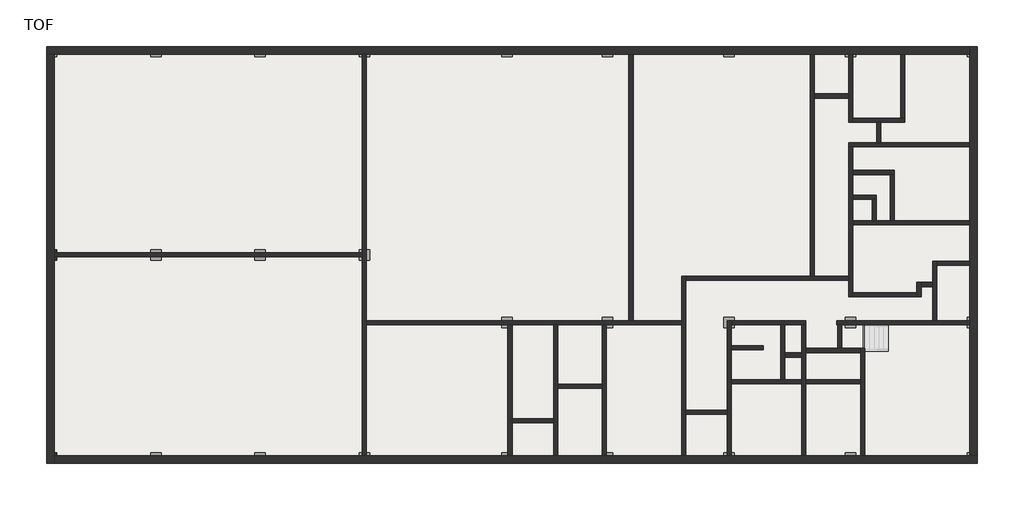
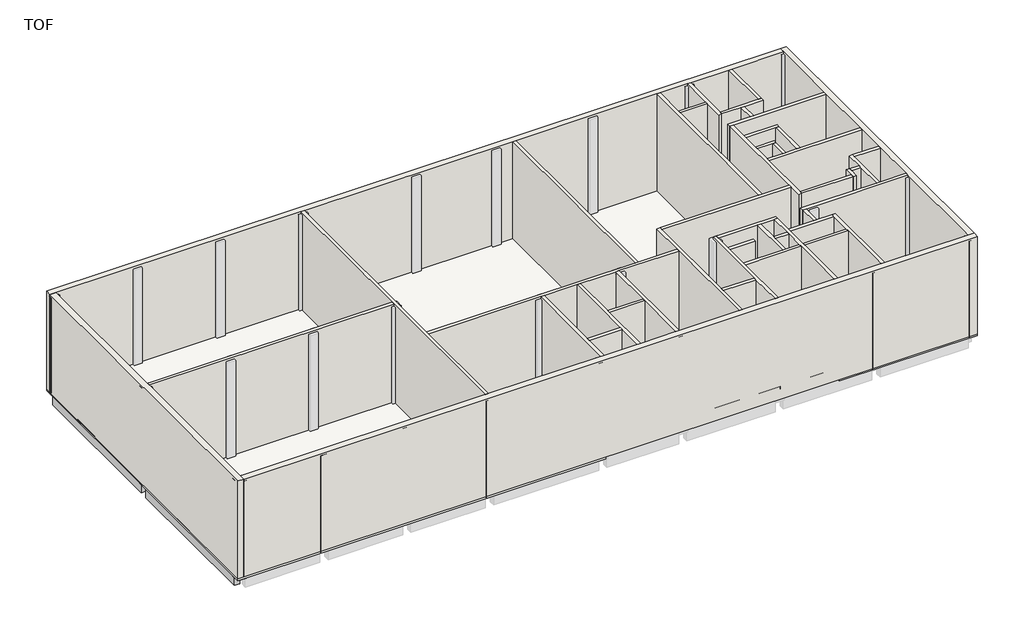
# One storey, part 1 of 2: 45 walls, 6 slabs, 2 beams, 2 columns.
"""IFC4 building model written with IfcOpenShell, lengths in millimetres."""

from ifc_helpers import new_model, si_unit, frame, origin, origin_with_axes, place, context, project, spatial, polyline, outline, extrude, faceted_brep, element, save

model = new_model("IFC4")

# Units and contexts
model_context = context("Model", 3, world=origin())
ifc_project = project(units=[si_unit("LENGTHUNIT", "METRE", prefix="MILLI")], contexts=[model_context])

# Site, building, storey
site = spatial("IfcSite", under=ifc_project)
building = spatial("IfcBuilding", under=site)
storey = spatial("IfcBuildingStorey", under=building, Name="TOF", Elevation=150.0)

# Beams
placement = place(None, origin())
element("IfcBeam", 1, ObjectType="RC Beam_Rectangular : H_SB_ACB_B400xH900", at=placement, inside=storey, context=model_context, shape_type="SweptSolid", body=[
    extrude(outline(polyline([(124.7, 12616.5208589), (-275.3, 12616.5208589), (-275.3, 23716.5208589), (124.7, 23716.5208589), (124.7, 12616.5208589)])), frame((0.0, 0.0, -750.0), z_axis=(0.0, 0.0, 1.0), x_axis=(1.0, 0.0, 0.0)), (0.0, 0.0, 1.0), 900.0),
])
element("IfcBeam", 2, ObjectType="RC Beam_Rectangular : H_SB_ACB_B400xH900", at=placement, inside=storey, context=model_context, shape_type="SweptSolid", body=[
    extrude(outline(polyline([(124.7, 916.5208589), (-275.3, 916.5208589), (-275.3, 12016.5208589), (124.7, 12016.5208589), (124.7, 916.5208589)])), frame((0.0, 0.0, -750.0), z_axis=(0.0, 0.0, 1.0), x_axis=(1.0, 0.0, 0.0)), (0.0, 0.0, 1.0), 900.0),
])

# Columns
element("IfcColumn", 3, ObjectType="RC_Column_Rectangular : H_SC_ACC_W600xL600", at=placement, inside=storey, context=model_context, shape_type="Brep", body=[
    faceted_brep([(224.7, 12616.5208589, 0.0), (224.7, 12016.5208589, 0.0), (-375.3, 12016.5208589, 0.0), (-375.3, 12616.5208589, 0.0), (224.7, 12616.5208589, 50.0), (224.7, 12316.5208589, 50.0), (224.7, 12316.5208589, 200.0), (224.7, 12616.5208589, 200.0), (224.7, 12616.5208589, 7500.0), (224.7, 12516.5208589, 7500.0), (224.7, 12116.5208589, 7500.0), (224.7, 12016.5208589, 7500.0), (124.7, 12016.5208589, 7500.0), (-275.3, 12016.5208589, 7500.0), (-375.3, 12016.5208589, 7500.0), (-375.3, 12616.5208589, 7500.0), (-375.3, 12616.5208589, 200.0), (-375.3, 12316.5208589, 200.0), (-375.3, 12316.5208589, 50.0), (-375.3, 12616.5208589, 50.0), (-275.3, 12616.5208589, 7500.0), (124.7, 12616.5208589, 7500.0)], [[[0, 1, 2, 3]], [[1, 0, 4, 5, 6, 7, 8, 9, 10, 11]], [[2, 1, 11, 12, 13, 14]], [[3, 2, 14, 15, 16, 17, 18, 19]], [[15, 20, 21, 8, 7, 16]], [[11, 10, 9, 8, 21, 20, 15, 14, 13, 12]], [[18, 5, 4, 19]], [[6, 17, 16, 7]], [[5, 18, 17, 6]], [[0, 3, 19, 4]]]),
])
element("IfcColumn", 4, ObjectType="RC_Column_Rectangular : H_SC_ACC_W600xL600", at=placement, inside=storey, context=model_context, shape_type="Brep", body=[
    faceted_brep([(224.7, 916.5208589, 0.0), (224.7, 316.5208589, 0.0), (-375.3, 316.5208589, 0.0), (-375.3, 916.5208589, 0.0), (224.7, 916.5208589, 7500.0), (224.7, 816.5208589, 7500.0), (224.7, 416.5208589, 7500.0), (224.7, 316.5208589, 7500.0), (-375.3, 316.5208589, 7500.0), (-375.3, 916.5208589, 7500.0), (-275.3, 916.5208589, 7500.0), (124.7, 916.5208589, 7500.0)], [[[0, 1, 2, 3]], [[4, 5, 6, 7, 1, 0]], [[7, 8, 2, 1]], [[8, 9, 3, 2]], [[9, 10, 11, 4, 0, 3]], [[4, 11, 10, 9, 8, 7, 6, 5]]]),
])

# Slabs
element("IfcSlab", 5, ObjectType="H_FL_AMF_RC Slab_T150", at=placement, inside=storey, context=model_context, shape_type="Brep", body=[
    faceted_brep([(-375.3, 24316.5208589, 50.0), (224.7, 24316.5208589, 50.0), (5624.7, 24316.5208589, 50.0), (6224.7, 24316.5208589, 50.0), (11624.7, 24316.5208589, 50.0), (12224.7, 24316.5208589, 50.0), (17624.7, 24316.5208589, 50.0), (18224.7, 24316.5208589, 50.0), (25824.7, 24316.5208589, 50.0), (26424.7, 24316.5208589, 50.0), (31624.7, 24316.5208589, 50.0), (32224.7, 24316.5208589, 50.0), (38624.7, 24316.5208589, 50.0), (39224.7, 24316.5208589, 50.0), (43724.7, 24316.5208589, 50.0), (43724.7, 10966.5208589, 50.0), (36324.7, 10966.5208589, 50.0), (36324.7, 8416.5208589, 50.0), (32224.7, 8416.5208589, 50.0), (31624.7, 8416.5208589, 50.0), (26424.7, 8416.5208589, 50.0), (25824.7, 8416.5208589, 50.0), (17924.7, 8416.5208589, 50.0), (17924.7, 12016.5208589, 50.0), (17924.7, 12316.5208589, 50.0), (17624.7, 12316.5208589, 50.0), (12224.7, 12316.5208589, 50.0), (11624.7, 12316.5208589, 50.0), (6224.7, 12316.5208589, 50.0), (5624.7, 12316.5208589, 50.0), (224.7, 12316.5208589, 50.0), (-375.3, 12316.5208589, 50.0), (-375.3, 12616.5208589, 50.0), (-375.3, 23716.5208589, 50.0), (-375.3, 24316.5208589, 200.0), (-375.3, 23716.5208589, 200.0), (-375.3, 12616.5208589, 200.0), (-375.3, 12316.5208589, 200.0), (224.7, 12316.5208589, 200.0), (5624.7, 12316.5208589, 200.0), (6224.7, 12316.5208589, 200.0), (11624.7, 12316.5208589, 200.0), (12224.7, 12316.5208589, 200.0), (17624.7, 12316.5208589, 200.0), (17924.7, 12316.5208589, 200.0), (17924.7, 12016.5208589, 200.0), (17924.7, 8416.5208589, 200.0), (25824.7, 8416.5208589, 200.0), (26424.7, 8416.5208589, 200.0), (31624.7, 8416.5208589, 200.0), (32224.7, 8416.5208589, 200.0), (36324.7, 8416.5208589, 200.0), (36324.7, 10966.5208589, 200.0), (43724.7, 10966.5208589, 200.0), (43724.7, 24316.5208589, 200.0), (39224.7, 24316.5208589, 200.0), (38624.7, 24316.5208589, 200.0), (32224.7, 24316.5208589, 200.0), (31624.7, 24316.5208589, 200.0), (26424.7, 24316.5208589, 200.0), (25824.7, 24316.5208589, 200.0), (18224.7, 24316.5208589, 200.0), (17624.7, 24316.5208589, 200.0), (12224.7, 24316.5208589, 200.0), (11624.7, 24316.5208589, 200.0), (6224.7, 24316.5208589, 200.0), (5624.7, 24316.5208589, 200.0), (224.7, 24316.5208589, 200.0)], [[[0, 1, 2, 3, 4, 5, 6, 7, 8, 9, 10, 11, 12, 13, 14, 15, 16, 17, 18, 19, 20, 21, 22, 23, 24, 25, 26, 27, 28, 29, 30, 31, 32, 33]], [[34, 35, 36, 37, 38, 39, 40, 41, 42, 43, 44, 45, 46, 47, 48, 49, 50, 51, 52, 53, 54, 55, 56, 57, 58, 59, 60, 61, 62, 63, 64, 65, 66, 67]], [[0, 33, 32, 31, 37, 36, 35, 34]], [[14, 13, 12, 11, 10, 9, 8, 7, 6, 5, 4, 3, 2, 1, 0, 34, 67, 66, 65, 64, 63, 62, 61, 60, 59, 58, 57, 56, 55, 54]], [[15, 14, 54, 53]], [[16, 15, 53, 52]], [[17, 16, 52, 51]], [[22, 21, 20, 19, 18, 17, 51, 50, 49, 48, 47, 46]], [[24, 23, 22, 46, 45, 44]], [[31, 30, 29, 28, 27, 26, 25, 24, 44, 43, 42, 41, 40, 39, 38, 37]]]),
])
element("IfcSlab", 6, ObjectType="H_FL_AMF_RC Slab_T150", at=placement, inside=storey, context=model_context, shape_type="Brep", body=[
    faceted_brep([(53224.7, 11850.5208589, 1000.0), (50777.7, 11850.5208589, 1000.0), (50777.7, 8416.5208589, 1000.0), (46624.7, 8416.5208589, 1000.0), (46624.7, 5013.5208589, 1000.0), (43341.7, 5013.5208589, 1000.0), (43224.7, 5013.5208589, 1000.0), (43224.7, 8299.5208589, 1000.0), (43224.7, 8416.5208589, 1000.0), (39041.7, 8416.5208589, 1000.0), (38924.7, 8416.5208589, 1000.0), (38924.7, 746.5208589, 1000.0), (38924.7, 316.5208589, 1000.0), (26307.7, 316.5208589, 1000.0), (26307.7, 8416.5208589, 1000.0), (36324.7, 8416.5208589, 1000.0), (36324.7, 10966.5208589, 1000.0), (43724.7, 10966.5208589, 1000.0), (43724.7, 24316.5208589, 1000.0), (53224.7, 24316.5208589, 1000.0), (53224.7, 11850.5208589, 1150.0), (53224.7, 24316.5208589, 1150.0), (43724.7, 24316.5208589, 1150.0), (43724.7, 10966.5208589, 1150.0), (36324.7, 10966.5208589, 1150.0), (36324.7, 8416.5208589, 1150.0), (26307.7, 8416.5208589, 1150.0), (26307.7, 316.5208589, 1150.0), (38924.7, 316.5208589, 1150.0), (38924.7, 746.5208589, 1150.0), (38924.7, 8416.5208589, 1150.0), (39041.7, 8416.5208589, 1150.0), (43224.7, 8416.5208589, 1150.0), (43224.7, 8299.5208589, 1150.0), (43224.7, 5013.5208589, 1150.0), (43341.7, 5013.5208589, 1150.0), (46624.7, 5013.5208589, 1150.0), (46624.7, 8416.5208589, 1150.0), (50777.7, 8416.5208589, 1150.0), (50777.7, 11850.5208589, 1150.0)], [[[0, 1, 2, 3, 4, 5, 6, 7, 8, 9, 10, 11, 12, 13, 14, 15, 16, 17, 18, 19]], [[20, 21, 22, 23, 24, 25, 26, 27, 28, 29, 30, 31, 32, 33, 34, 35, 36, 37, 38, 39]], [[13, 12, 28, 27]], [[19, 18, 22, 21]], [[0, 19, 21, 20]], [[1, 0, 20, 39]], [[2, 1, 39, 38]], [[3, 2, 38, 37]], [[4, 3, 37, 36]], [[6, 5, 4, 36, 35, 34]], [[8, 7, 6, 34, 33, 32]], [[10, 9, 8, 32, 31, 30]], [[12, 11, 10, 30, 29, 28]], [[14, 13, 27, 26]], [[15, 14, 26, 25]], [[16, 15, 25, 24]], [[17, 16, 24, 23]], [[18, 17, 23, 22]]]),
])
element("IfcSlab", 7, ObjectType="H_FL_AMF_RC Slab_T150", at=placement, inside=storey, context=model_context, shape_type="SweptSolid", body=[
    extrude(outline(polyline([(17924.7, 12316.5208589), (17924.7, 8416.5208589), (26307.7, 8416.5208589), (26307.7, 316.5208589), (-375.3, 316.5208589), (-375.3, 12316.5208589), (17924.7, 12316.5208589)])), origin_with_axes(), (0.0, 0.0, 1.0), 150.0),
])
element("IfcSlab", 8, ObjectType="H_FL_AMF_RC Slab_T150", at=placement, inside=storey, context=model_context, shape_type="SweptSolid", body=[
    extrude(outline(polyline([(53224.7, 11850.5208589), (53224.7, 8416.5208589), (50777.7, 8416.5208589), (50777.7, 11850.5208589), (53224.7, 11850.5208589)])), frame((0.0, 0.0, 1000.0), z_axis=(0.0, 0.0, 1.0), x_axis=(1.0, 0.0, 0.0)), (0.0, 0.0, 1.0), 150.0),
])
element("IfcSlab", 9, ObjectType="H_FL_AMF_RC Slab_T150", at=placement, inside=storey, context=model_context, shape_type="SweptSolid", body=[
    extrude(outline(polyline([(46624.7, 8416.5208589), (53224.7, 8416.5208589), (53224.7, 316.5208589), (43224.7, 316.5208589), (43224.7, 5018.5208589), (46624.7, 5018.5208589), (46624.7, 8416.5208589)])), frame((0.0, 0.0, 50.0), z_axis=(0.0, 0.0, 1.0), x_axis=(1.0, 0.0, 0.0)), (0.0, 0.0, 1.0), 150.0),
])
element("IfcSlab", 10, ObjectType="H_FL_AMF_RC Slab_T150", at=placement, inside=storey, context=model_context, shape_type="SweptSolid", body=[
    extrude(outline(polyline([(38924.7, 316.5208589), (38924.7, 8416.5208589), (43224.7, 8416.5208589), (43224.7, 316.5208589), (38924.7, 316.5208589)])), frame((0.0, 0.0, 950.0), z_axis=(0.0, 0.0, 1.0), x_axis=(1.0, 0.0, 0.0)), (0.0, 0.0, 1.0), 150.0),
])

# Walls
element("IfcWall", 11, ObjectType="H_WA_AMW_Brick Wall_Ext (0.5B_50_1.0B / Emulsion)", at=placement, inside=storey, context=model_context, shape_type="Brep", body=[
    faceted_brep([(-375.3, 23886.5208589, 150.0), (54.7, 23886.5208589, 150.0), (17807.7, 23886.5208589, 150.0), (18041.7, 23886.5208589, 150.0), (33157.7, 23886.5208589, 150.0), (33391.7, 23886.5208589, 150.0), (43607.7, 23886.5208589, 150.0), (43841.7, 23886.5208589, 150.0), (52794.7, 23886.5208589, 150.0), (52794.7, 23886.5208589, 7650.0), (49041.7, 23886.5208589, 7650.0), (48807.7, 23886.5208589, 7650.0), (46041.7, 23886.5208589, 7650.0), (45807.7, 23886.5208589, 7650.0), (43841.7, 23886.5208589, 7650.0), (43607.7, 23886.5208589, 7650.0), (33391.7, 23886.5208589, 7650.0), (33157.7, 23886.5208589, 7650.0), (18041.7, 23886.5208589, 7650.0), (17807.7, 23886.5208589, 7650.0), (54.7, 23886.5208589, 7650.0), (-375.3, 23886.5208589, 7650.0), (-375.3, 24316.5208589, 150.0), (-375.3, 24316.5208589, 7650.0), (52794.7, 24316.5208589, 7650.0), (52794.7, 24316.5208589, 150.0)], [[[0, 1, 2, 3, 4, 5, 6, 7, 8, 9, 10, 11, 12, 13, 14, 15, 16, 17, 18, 19, 20, 21]], [[22, 23, 24, 25]], [[8, 7, 6, 5, 4, 3, 2, 1, 0, 22, 25]], [[21, 20, 19, 18, 17, 16, 15, 14, 13, 12, 11, 10, 9, 24, 23]], [[0, 21, 23, 22]], [[9, 8, 25, 24]]]),
])
element("IfcWall", 12, ObjectType="H_WA_AMW_Brick Wall_Ext (0.5B_50_1.0B / Emulsion)", at=placement, inside=storey, context=model_context, shape_type="Brep", body=[
    faceted_brep([(54.7, 316.5208589, 150.0), (54.7, 746.5208589, 150.0), (54.7, 12199.5208589, 150.0), (54.7, 12433.5208589, 150.0), (54.7, 23886.5208589, 150.0), (54.7, 23886.5208589, 7650.0), (54.7, 12433.5208589, 7650.0), (54.7, 12199.5208589, 7650.0), (54.7, 746.5208589, 7650.0), (54.7, 316.5208589, 7650.0), (-375.3, 316.5208589, 150.0), (-375.3, 316.5208589, 7650.0), (-375.3, 23886.5208589, 7650.0), (-375.3, 23886.5208589, 150.0)], [[[0, 1, 2, 3, 4, 5, 6, 7, 8, 9]], [[10, 11, 12, 13]], [[4, 3, 2, 1, 0, 10, 13]], [[9, 8, 7, 6, 5, 12, 11]], [[0, 9, 11, 10]], [[5, 4, 13, 12]]]),
])
element("IfcWall", 13, ObjectType="H_WA_AMW_Brick Wall_Ext (0.5B_50_1.0B / Emulsion)", at=placement, inside=storey, context=model_context, shape_type="Brep", body=[
    faceted_brep([(53224.7, 746.5208589, 150.0), (52794.7, 746.5208589, 150.0), (46741.7, 746.5208589, 150.0), (46507.7, 746.5208589, 150.0), (43341.7, 746.5208589, 150.0), (43107.7, 746.5208589, 150.0), (39041.7, 746.5208589, 150.0), (38807.7, 746.5208589, 150.0), (26424.7, 746.5208589, 150.0), (26190.7, 746.5208589, 150.0), (18041.7, 746.5208589, 150.0), (17807.7, 746.5208589, 150.0), (54.7, 746.5208589, 150.0), (54.7, 746.5208589, 7650.0), (17807.7, 746.5208589, 7650.0), (18041.7, 746.5208589, 7650.0), (26190.7, 746.5208589, 7650.0), (26424.7, 746.5208589, 7650.0), (28824.7, 746.5208589, 7650.0), (29058.7, 746.5208589, 7650.0), (31624.7, 746.5208589, 7650.0), (31858.7, 746.5208589, 7650.0), (36207.7, 746.5208589, 7650.0), (36441.7, 746.5208589, 7650.0), (38807.7, 746.5208589, 7650.0), (39041.7, 746.5208589, 7650.0), (43107.7, 746.5208589, 7650.0), (43341.7, 746.5208589, 7650.0), (46507.7, 746.5208589, 7650.0), (46741.7, 746.5208589, 7650.0), (52794.7, 746.5208589, 7650.0), (53224.7, 746.5208589, 7650.0), (53224.7, 316.5208589, 150.0), (53224.7, 316.5208589, 7650.0), (54.7, 316.5208589, 7650.0), (54.7, 316.5208589, 150.0)], [[[0, 1, 2, 3, 4, 5, 6, 7, 8, 9, 10, 11, 12, 13, 14, 15, 16, 17, 18, 19, 20, 21, 22, 23, 24, 25, 26, 27, 28, 29, 30, 31]], [[32, 33, 34, 35]], [[12, 11, 10, 9, 8, 7, 6, 5, 4, 3, 2, 1, 0, 32, 35]], [[31, 30, 29, 28, 27, 26, 25, 24, 23, 22, 21, 20, 19, 18, 17, 16, 15, 14, 13, 34, 33]], [[0, 31, 33, 32]], [[13, 12, 35, 34]]]),
])
element("IfcWall", 14, ObjectType="H_WA_AMW_Brick Wall_Ext (0.5B_50_1.0B / Emulsion)", at=placement, inside=storey, context=model_context, shape_type="Brep", body=[
    faceted_brep([(52794.7, 24316.5208589, 150.0), (52794.7, 23886.5208589, 150.0), (52794.7, 8533.5208589, 150.0), (52794.7, 8299.5208589, 150.0), (52794.7, 746.5208589, 150.0), (52794.7, 746.5208589, 7650.0), (52794.7, 8299.5208589, 7650.0), (52794.7, 8533.5208589, 7650.0), (52794.7, 11733.5208589, 7650.0), (52794.7, 11967.5208589, 7650.0), (52794.7, 14049.5208589, 7650.0), (52794.7, 14283.5208589, 7650.0), (52794.7, 18549.5208589, 7650.0), (52794.7, 18783.5208589, 7650.0), (52794.7, 23886.5208589, 7650.0), (52794.7, 24316.5208589, 7650.0), (53224.7, 24316.5208589, 150.0), (53224.7, 24316.5208589, 7650.0), (53224.7, 746.5208589, 7650.0), (53224.7, 746.5208589, 150.0)], [[[0, 1, 2, 3, 4, 5, 6, 7, 8, 9, 10, 11, 12, 13, 14, 15]], [[16, 17, 18, 19]], [[4, 3, 2, 1, 0, 16, 19]], [[15, 14, 13, 12, 11, 10, 9, 8, 7, 6, 5, 18, 17]], [[0, 15, 17, 16]], [[5, 4, 19, 18]]]),
])
element("IfcWall", 15, ObjectType="H_WA_AMW_Block Wall_Int_T200 (Both Plaster_Emulsion)", at=placement, inside=storey, context=model_context, shape_type="SweptSolid", body=[
    extrude(outline(polyline([(17807.7, 12199.5208589), (54.7, 12199.5208589), (54.7, 12433.5208589), (17807.7, 12433.5208589), (17807.7, 12199.5208589)])), frame((0.0, 0.0, 150.0), z_axis=(0.0, 0.0, 1.0), x_axis=(1.0, 0.0, 0.0)), (0.0, 0.0, 1.0), 7500.0),
])
element("IfcWall", 16, ObjectType="H_WA_AMW_Block Wall_Int_T200 (Both Plaster_Emulsion)", at=placement, inside=storey, context=model_context, shape_type="Brep", body=[
    faceted_brep([(17807.7, 23886.5208589, 150.0), (17807.7, 12433.5208589, 150.0), (17807.7, 12199.5208589, 150.0), (17807.7, 746.5208589, 150.0), (17807.7, 746.5208589, 7650.0), (17807.7, 12199.5208589, 7650.0), (17807.7, 12433.5208589, 7650.0), (17807.7, 23886.5208589, 7650.0), (18041.7, 23886.5208589, 150.0), (18041.7, 23886.5208589, 7650.0), (18041.7, 8533.5208589, 7650.0), (18041.7, 8299.5208589, 7650.0), (18041.7, 746.5208589, 7650.0), (18041.7, 746.5208589, 150.0), (18041.7, 8299.5208589, 150.0), (18041.7, 8533.5208589, 150.0)], [[[0, 1, 2, 3, 4, 5, 6, 7]], [[8, 9, 10, 11, 12, 13, 14, 15]], [[3, 2, 1, 0, 8, 15, 14, 13]], [[7, 6, 5, 4, 12, 11, 10, 9]], [[0, 7, 9, 8]], [[4, 3, 13, 12]]]),
])
element("IfcWall", 17, ObjectType="H_WA_AMW_Block Wall_Int_T200 (Both Plaster_Emulsion)", at=placement, inside=storey, context=model_context, shape_type="SweptSolid", body=[
    extrude(outline(polyline([(33157.7, 8533.5208589), (33157.7, 23886.5208589), (33391.7, 23886.5208589), (33391.7, 8533.5208589), (33157.7, 8533.5208589)])), frame((0.0, 0.0, 150.0), z_axis=(0.0, 0.0, 1.0), x_axis=(1.0, 0.0, 0.0)), (0.0, 0.0, 1.0), 7500.0),
])
element("IfcWall", 18, ObjectType="H_WA_AMW_Block Wall_Int_T200 (Both Plaster_Emulsion)", at=placement, inside=storey, context=model_context, shape_type="Brep", body=[
    faceted_brep([(18041.7, 8299.5208589, 150.0), (26190.7, 8299.5208589, 150.0), (26424.7, 8299.5208589, 150.0), (36207.7, 8299.5208589, 150.0), (36207.7, 8299.5208589, 7650.0), (31858.7, 8299.5208589, 7650.0), (31624.7, 8299.5208589, 7650.0), (29058.7, 8299.5208589, 7650.0), (28824.7, 8299.5208589, 7650.0), (26424.7, 8299.5208589, 7650.0), (26190.7, 8299.5208589, 7650.0), (18041.7, 8299.5208589, 7650.0), (36207.7, 8533.5208589, 150.0), (33391.7, 8533.5208589, 150.0), (33157.7, 8533.5208589, 150.0), (18041.7, 8533.5208589, 150.0), (18041.7, 8533.5208589, 7650.0), (33157.7, 8533.5208589, 7650.0), (33391.7, 8533.5208589, 7650.0), (36207.7, 8533.5208589, 7650.0)], [[[0, 1, 2, 3, 4, 5, 6, 7, 8, 9, 10, 11]], [[12, 13, 14, 15, 16, 17, 18, 19]], [[3, 2, 1, 0, 15, 14, 13, 12]], [[11, 10, 9, 8, 7, 6, 5, 4, 19, 18, 17, 16]], [[0, 11, 16, 15]], [[4, 3, 12, 19]]]),
])
element("IfcWall", 19, ObjectType="H_WA_AMW_Block Wall_Int_T200 (Both Plaster_Emulsion)", at=placement, inside=storey, context=model_context, shape_type="Brep", body=[
    faceted_brep([(36207.7, 11083.5208589, 1150.0), (36207.7, 746.5208589, 1150.0), (36207.7, 746.5208589, 7650.0), (36207.7, 8299.5208589, 7650.0), (36207.7, 8533.5208589, 7650.0), (36207.7, 11083.5208589, 7650.0), (36441.7, 11083.5208589, 1150.0), (36441.7, 11083.5208589, 7650.0), (36441.7, 10849.5208589, 7650.0), (36441.7, 3380.5208589, 7650.0), (36441.7, 3146.5208589, 7650.0), (36441.7, 746.5208589, 7650.0), (36441.7, 746.5208589, 1150.0), (36441.7, 3146.5208589, 1150.0), (36441.7, 3380.5208589, 1150.0)], [[[0, 1, 2, 3, 4, 5]], [[6, 7, 8, 9, 10, 11, 12, 13, 14]], [[1, 0, 6, 14, 13, 12]], [[5, 4, 3, 2, 11, 10, 9, 8, 7]], [[2, 1, 12, 11]], [[0, 5, 7, 6]]]),
])
element("IfcWall", 20, ObjectType="H_WA_AMW_Block Wall_Int_T200 (Both Plaster_Emulsion)", at=placement, inside=storey, context=model_context, shape_type="Brep", body=[
    faceted_brep([(36441.7, 10849.5208589, 150.0), (45807.7, 10849.5208589, 150.0), (45807.7, 10849.5208589, 7650.0), (36441.7, 10849.5208589, 7650.0), (45807.7, 11083.5208589, 150.0), (43841.7, 11083.5208589, 150.0), (43607.7, 11083.5208589, 150.0), (36441.7, 11083.5208589, 150.0), (36441.7, 11083.5208589, 1150.0), (36441.7, 11083.5208589, 7650.0), (43607.7, 11083.5208589, 7650.0), (43841.7, 11083.5208589, 7650.0), (45807.7, 11083.5208589, 7650.0)], [[[0, 1, 2, 3]], [[4, 5, 6, 7, 8, 9, 10, 11, 12]], [[1, 0, 7, 6, 5, 4]], [[3, 2, 12, 11, 10, 9]], [[0, 3, 9, 8, 7]], [[2, 1, 4, 12]]]),
])
element("IfcWall", 21, ObjectType="H_WA_AMW_Block Wall_Int_T200 (Both Plaster_Emulsion)", at=placement, inside=storey, context=model_context, shape_type="Brep", body=[
    faceted_brep([(43841.7, 11083.5208589, 150.0), (43841.7, 23886.5208589, 150.0), (43841.7, 23886.5208589, 7650.0), (43841.7, 21586.5208589, 7650.0), (43841.7, 21352.5208589, 7650.0), (43841.7, 11083.5208589, 7650.0), (43607.7, 23886.5208589, 150.0), (43607.7, 11083.5208589, 150.0), (43607.7, 11083.5208589, 7650.0), (43607.7, 23886.5208589, 7650.0)], [[[0, 1, 2, 3, 4, 5]], [[6, 7, 8, 9]], [[1, 0, 7, 6]], [[5, 4, 3, 2, 9, 8]], [[2, 1, 6, 9]], [[0, 5, 8, 7]]]),
])
element("IfcWall", 22, ObjectType="H_WA_AMW_Block Wall_Int_T200 (Both Plaster_Emulsion)", at=placement, inside=storey, context=model_context, shape_type="SweptSolid", body=[
    extrude(outline(polyline([(45807.7, 21352.5208589), (43841.7, 21352.5208589), (43841.7, 21586.5208589), (45807.7, 21586.5208589), (45807.7, 21352.5208589)])), frame((0.0, 0.0, 1150.0), z_axis=(0.0, 0.0, 1.0), x_axis=(1.0, 0.0, 0.0)), (0.0, 0.0, 1.0), 6500.0),
])
element("IfcWall", 23, ObjectType="H_WA_AMW_Block Wall_Int_T200 (Both Plaster_Emulsion)", at=placement, inside=storey, context=model_context, shape_type="Brep", body=[
    faceted_brep([(45807.7, 23886.5208589, 1150.0), (45807.7, 21586.5208589, 1150.0), (45807.7, 21352.5208589, 1150.0), (45807.7, 19949.5208589, 1150.0), (45807.7, 19949.5208589, 7650.0), (45807.7, 21352.5208589, 7650.0), (45807.7, 21586.5208589, 7650.0), (45807.7, 23886.5208589, 7650.0), (46041.7, 23886.5208589, 1150.0), (46041.7, 23886.5208589, 7650.0), (46041.7, 20183.5208589, 7650.0), (46041.7, 19949.5208589, 7650.0), (46041.7, 19949.5208589, 1150.0), (46041.7, 20183.5208589, 1150.0)], [[[0, 1, 2, 3, 4, 5, 6, 7]], [[8, 9, 10, 11, 12, 13]], [[3, 2, 1, 0, 8, 13, 12]], [[7, 6, 5, 4, 11, 10, 9]], [[0, 7, 9, 8]], [[4, 3, 12, 11]]]),
])
element("IfcWall", 24, ObjectType="H_WA_AMW_Block Wall_Int_T200 (Both Plaster_Emulsion)", at=placement, inside=storey, context=model_context, shape_type="SweptSolid", body=[
    extrude(outline(polyline([(49743.7, 9899.5208589), (46041.7, 9899.5208589), (46041.7, 10133.5208589), (49743.7, 10133.5208589), (49743.7, 9899.5208589)])), frame((0.0, 0.0, 1150.0), z_axis=(0.0, 0.0, 1.0), x_axis=(1.0, 0.0, 0.0)), (0.0, 0.0, 1.0), 6500.0),
])
element("IfcWall", 25, ObjectType="H_WA_AMW_Block Wall_Int_T200 (Both Plaster_Emulsion)", at=placement, inside=storey, context=model_context, shape_type="Brep", body=[
    faceted_brep([(50660.7, 11967.5208589, 150.0), (50660.7, 8533.5208589, 150.0), (50660.7, 8533.5208589, 7650.0), (50660.7, 10499.5208589, 7650.0), (50660.7, 10733.5208589, 7650.0), (50660.7, 11967.5208589, 7650.0), (50894.7, 8533.5208589, 150.0), (50894.7, 11967.5208589, 150.0), (50894.7, 11967.5208589, 1150.0), (50894.7, 11967.5208589, 7650.0), (50894.7, 11733.5208589, 7650.0), (50894.7, 8533.5208589, 7650.0)], [[[0, 1, 2, 3, 4, 5]], [[6, 7, 8, 9, 10, 11]], [[1, 0, 7, 6]], [[5, 4, 3, 2, 11, 10, 9]], [[0, 5, 9, 8, 7]], [[2, 1, 6, 11]]]),
])
element("IfcWall", 26, ObjectType="H_WA_AMW_Block Wall_Int_T200 (Both Plaster_Emulsion)", at=placement, inside=storey, context=model_context, shape_type="SweptSolid", body=[
    extrude(outline(polyline([(52794.7, 11733.5208589), (50894.7, 11733.5208589), (50894.7, 11967.5208589), (52794.7, 11967.5208589), (52794.7, 11733.5208589)])), frame((0.0, 0.0, 1150.0), z_axis=(0.0, 0.0, 1.0), x_axis=(1.0, 0.0, 0.0)), (0.0, 0.0, 1.0), 6500.0),
])
element("IfcWall", 27, ObjectType="H_WA_AMW_Block Wall_Int_T200 (Both Plaster_Emulsion)", at=placement, inside=storey, context=model_context, shape_type="Brep", body=[
    faceted_brep([(49977.7, 9899.5208589, 1150.0), (49977.7, 10499.5208589, 1150.0), (49977.7, 10733.5208589, 1150.0), (49977.7, 10733.5208589, 7650.0), (49977.7, 10499.5208589, 7650.0), (49977.7, 9899.5208589, 7650.0), (49743.7, 9899.5208589, 1150.0), (49743.7, 9899.5208589, 7650.0), (49743.7, 10133.5208589, 7650.0), (49743.7, 10733.5208589, 7650.0), (49743.7, 10733.5208589, 1150.0), (49743.7, 10133.5208589, 1150.0)], [[[0, 1, 2, 3, 4, 5]], [[6, 7, 8, 9, 10, 11]], [[2, 1, 0, 6, 11, 10]], [[5, 4, 3, 9, 8, 7]], [[3, 2, 10, 9]], [[0, 5, 7, 6]]]),
])
element("IfcWall", 28, ObjectType="H_WA_AMW_Block Wall_Int_T200 (Both Plaster_Emulsion)", at=placement, inside=storey, context=model_context, shape_type="SweptSolid", body=[
    extrude(outline(polyline([(50660.7, 10499.5208589), (49977.7, 10499.5208589), (49977.7, 10733.5208589), (50660.7, 10733.5208589), (50660.7, 10499.5208589)])), frame((0.0, 0.0, 1150.0), z_axis=(0.0, 0.0, 1.0), x_axis=(1.0, 0.0, 0.0)), (0.0, 0.0, 1.0), 6500.0),
])
element("IfcWall", 29, ObjectType="H_WA_AMW_Block Wall_Int_T200 (Both Plaster_Emulsion)", at=placement, inside=storey, context=model_context, shape_type="Brep", body=[
    faceted_brep([(46507.7, 6933.5208589, 150.0), (46507.7, 6699.5208589, 150.0), (46507.7, 5130.5208589, 150.0), (46507.7, 4896.5208589, 150.0), (46507.7, 746.5208589, 150.0), (46507.7, 746.5208589, 7650.0), (46507.7, 4896.5208589, 7650.0), (46507.7, 5130.5208589, 7650.0), (46507.7, 6699.5208589, 7650.0), (46507.7, 6933.5208589, 7650.0), (46741.7, 6933.5208589, 150.0), (46741.7, 6933.5208589, 7650.0), (46741.7, 746.5208589, 7650.0), (46741.7, 746.5208589, 150.0)], [[[0, 1, 2, 3, 4, 5, 6, 7, 8, 9]], [[10, 11, 12, 13]], [[4, 3, 2, 1, 0, 10, 13]], [[9, 8, 7, 6, 5, 12, 11]], [[5, 4, 13, 12]], [[0, 9, 11, 10]]]),
])
element("IfcWall", 30, ObjectType="H_WA_AMW_Block Wall_Int_T200 (Both Plaster_Emulsion)", at=placement, inside=storey, context=model_context, shape_type="Brep", body=[
    faceted_brep([(43341.7, 6699.5208589, 150.0), (46507.7, 6699.5208589, 150.0), (46507.7, 6699.5208589, 7650.0), (43341.7, 6699.5208589, 7650.0), (46507.7, 6933.5208589, 150.0), (45409.8778017, 6933.5208589, 150.0), (45175.8778017, 6933.5208589, 150.0), (43341.7, 6933.5208589, 150.0), (43341.7, 6933.5208589, 7650.0), (45175.8778017, 6933.5208589, 7650.0), (45409.8778017, 6933.5208589, 7650.0), (46507.7, 6933.5208589, 7650.0)], [[[0, 1, 2, 3]], [[4, 5, 6, 7, 8, 9, 10, 11]], [[1, 0, 7, 6, 5, 4]], [[3, 2, 11, 10, 9, 8]], [[2, 1, 4, 11]], [[0, 3, 8, 7]]]),
])
element("IfcWall", 31, ObjectType="H_WA_AMW_Block Wall_Int_T200 (Both Plaster_Emulsion)", at=placement, inside=storey, context=model_context, shape_type="Brep", body=[
    faceted_brep([(52794.7, 8533.5208589, 150.0), (50894.7, 8533.5208589, 150.0), (50660.7, 8533.5208589, 150.0), (45124.7, 8533.5208589, 150.0), (45124.7, 8533.5208589, 7650.0), (50660.7, 8533.5208589, 7650.0), (50894.7, 8533.5208589, 7650.0), (52794.7, 8533.5208589, 7650.0), (52794.7, 8299.5208589, 150.0), (52794.7, 8299.5208589, 7650.0), (45409.8778017, 8299.5208589, 7650.0), (45175.8778017, 8299.5208589, 7650.0), (45124.7, 8299.5208589, 7650.0), (45124.7, 8299.5208589, 150.0), (45175.8778017, 8299.5208589, 150.0), (45409.8778017, 8299.5208589, 150.0)], [[[0, 1, 2, 3, 4, 5, 6, 7]], [[8, 9, 10, 11, 12, 13, 14, 15]], [[3, 2, 1, 0, 8, 15, 14, 13]], [[4, 3, 13, 12]], [[7, 6, 5, 4, 12, 11, 10, 9]], [[0, 7, 9, 8]]]),
])
element("IfcWall", 32, ObjectType="H_WA_AMW_Block Wall_Int_T200 (Both Plaster_Emulsion)", at=placement, inside=storey, context=model_context, shape_type="Brep", body=[
    faceted_brep([(38807.7, 8533.5208589, 150.0), (38807.7, 746.5208589, 150.0), (38807.7, 746.5208589, 1000.0), (38807.7, 8533.5208589, 1000.0), (38807.7, 746.5208589, 7650.0), (38807.7, 3146.5208589, 7650.0), (38807.7, 3380.5208589, 7650.0), (38807.7, 8533.5208589, 7650.0), (38807.7, 8533.5208589, 1150.0), (38807.7, 3380.5208589, 1150.0), (38807.7, 3146.5208589, 1150.0), (38807.7, 746.5208589, 1150.0), (39041.7, 746.5208589, 150.0), (39041.7, 4896.5208589, 150.0), (39041.7, 5130.5208589, 150.0), (39041.7, 6846.5208589, 150.0), (39041.7, 7080.5208589, 150.0), (39041.7, 8299.5208589, 150.0), (39041.7, 8533.5208589, 150.0), (39041.7, 8533.5208589, 1000.0), (39041.7, 8416.5208589, 1000.0), (39041.7, 8416.5208589, 1150.0), (39041.7, 8533.5208589, 1150.0), (39041.7, 8533.5208589, 7650.0), (39041.7, 8299.5208589, 7650.0), (39041.7, 7080.5208589, 7650.0), (39041.7, 6846.5208589, 7650.0), (39041.7, 5130.5208589, 7650.0), (39041.7, 4896.5208589, 7650.0), (39041.7, 746.5208589, 7650.0), (38924.7, 746.5208589, 1150.0), (38924.7, 746.5208589, 1000.0), (38924.7, 8416.5208589, 1000.0), (38924.7, 8416.5208589, 1150.0)], [[[0, 1, 2, 3]], [[4, 5, 6, 7, 8, 9, 10, 11]], [[12, 13, 14, 15, 16, 17, 18, 19, 20, 21, 22, 23, 24, 25, 26, 27, 28, 29]], [[1, 0, 18, 17, 16, 15, 14, 13, 12]], [[7, 6, 5, 4, 29, 28, 27, 26, 25, 24, 23]], [[1, 12, 29, 4, 11, 30, 31, 2]], [[7, 23, 22, 8]], [[18, 0, 3, 19]], [[31, 32, 20, 19, 3, 2]], [[21, 33, 30, 11, 10, 9, 8, 22]], [[32, 33, 21, 20]], [[33, 32, 31, 30]]]),
])
element("IfcWall", 33, ObjectType="H_WA_AMW_Block Wall_Int_T200 (Both Plaster_Emulsion)", at=placement, inside=storey, context=model_context, shape_type="Brep", body=[
    faceted_brep([(39041.7, 8299.5208589, 150.0), (41890.7, 8299.5208589, 150.0), (42124.7, 8299.5208589, 150.0), (43107.7, 8299.5208589, 150.0), (43341.7, 8299.5208589, 150.0), (43341.7, 8299.5208589, 1000.0), (43224.7, 8299.5208589, 1000.0), (43224.7, 8299.5208589, 1150.0), (43341.7, 8299.5208589, 1150.0), (43341.7, 8299.5208589, 7650.0), (43107.7, 8299.5208589, 7650.0), (42124.7, 8299.5208589, 7650.0), (41890.7, 8299.5208589, 7650.0), (39041.7, 8299.5208589, 7650.0), (43341.7, 8533.5208589, 150.0), (39041.7, 8533.5208589, 150.0), (39041.7, 8533.5208589, 1000.0), (43341.7, 8533.5208589, 1000.0), (39041.7, 8533.5208589, 7650.0), (43341.7, 8533.5208589, 7650.0), (43341.7, 8533.5208589, 1150.0), (39041.7, 8533.5208589, 1150.0), (39041.7, 8416.5208589, 1150.0), (39041.7, 8416.5208589, 1000.0), (43224.7, 8416.5208589, 1000.0), (43224.7, 8416.5208589, 1150.0)], [[[0, 1, 2, 3, 4, 5, 6, 7, 8, 9, 10, 11, 12, 13]], [[14, 15, 16, 17]], [[18, 19, 20, 21]], [[4, 3, 2, 1, 0, 15, 14]], [[13, 12, 11, 10, 9, 19, 18]], [[0, 13, 18, 21, 22, 23, 16, 15]], [[4, 14, 17, 5]], [[19, 9, 8, 20]], [[23, 24, 6, 5, 17, 16]], [[7, 25, 22, 21, 20, 8]], [[24, 25, 7, 6]], [[25, 24, 23, 22]]]),
])
element("IfcWall", 34, ObjectType="H_WA_AMW_Block Wall_Int_T200 (Both Plaster_Emulsion)", at=placement, inside=storey, context=model_context, shape_type="Brep", body=[
    faceted_brep([(43107.7, 8299.5208589, 150.0), (43107.7, 6673.5208589, 150.0), (43107.7, 6439.5208589, 150.0), (43107.7, 5130.5208589, 150.0), (43107.7, 4896.5208589, 150.0), (43107.7, 746.5208589, 150.0), (43107.7, 746.5208589, 7650.0), (43107.7, 4896.5208589, 7650.0), (43107.7, 5130.5208589, 7650.0), (43107.7, 6439.5208589, 7650.0), (43107.7, 6673.5208589, 7650.0), (43107.7, 8299.5208589, 7650.0), (43341.7, 746.5208589, 150.0), (43341.7, 4896.5208589, 150.0), (43341.7, 5130.5208589, 150.0), (43341.7, 6699.5208589, 150.0), (43341.7, 6933.5208589, 150.0), (43341.7, 8299.5208589, 150.0), (43341.7, 8299.5208589, 1000.0), (43341.7, 5013.5208589, 1000.0), (43341.7, 5013.5208589, 1150.0), (43341.7, 8299.5208589, 1150.0), (43341.7, 8299.5208589, 7650.0), (43341.7, 6933.5208589, 7650.0), (43341.7, 6699.5208589, 7650.0), (43341.7, 5130.5208589, 7650.0), (43341.7, 4896.5208589, 7650.0), (43341.7, 746.5208589, 7650.0), (43224.7, 8299.5208589, 1150.0), (43224.7, 8299.5208589, 1000.0), (43224.7, 5013.5208589, 1000.0), (43224.7, 5013.5208589, 1150.0)], [[[0, 1, 2, 3, 4, 5, 6, 7, 8, 9, 10, 11]], [[12, 13, 14, 15, 16, 17, 18, 19, 20, 21, 22, 23, 24, 25, 26, 27]], [[5, 4, 3, 2, 1, 0, 17, 16, 15, 14, 13, 12]], [[11, 10, 9, 8, 7, 6, 27, 26, 25, 24, 23, 22]], [[0, 11, 22, 21, 28, 29, 18, 17]], [[6, 5, 12, 27]], [[29, 30, 19, 18]], [[20, 31, 28, 21]], [[30, 31, 20, 19]], [[31, 30, 29, 28]]]),
])
element("IfcWall", 35, ObjectType="H_WA_AMW_Block Wall_Int_T200 (Both Plaster_Emulsion)", at=placement, inside=storey, context=model_context, shape_type="Brep", body=[
    faceted_brep([(39041.7, 4896.5208589, 7650.0), (39041.7, 4896.5208589, 150.0), (43107.7, 4896.5208589, 150.0), (43107.7, 4896.5208589, 7650.0), (39041.7, 5130.5208589, 150.0), (39041.7, 5130.5208589, 7650.0), (41890.7, 5130.5208589, 7650.0), (42124.7, 5130.5208589, 7650.0), (43107.7, 5130.5208589, 7650.0), (43107.7, 5130.5208589, 150.0), (42124.7, 5130.5208589, 150.0), (41890.7, 5130.5208589, 150.0)], [[[0, 1, 2, 3]], [[4, 5, 6, 7, 8, 9, 10, 11]], [[1, 4, 11, 10, 9, 2]], [[5, 0, 3, 8, 7, 6]], [[1, 0, 5, 4]], [[3, 2, 9, 8]]]),
    faceted_brep([(46507.7, 4896.5208589, 150.0), (46507.7, 4896.5208589, 7650.0), (43341.7, 4896.5208589, 7650.0), (43341.7, 4896.5208589, 150.0), (46507.7, 5130.5208589, 7650.0), (46507.7, 5130.5208589, 150.0), (43341.7, 5130.5208589, 150.0), (43341.7, 5130.5208589, 7650.0)], [[[0, 1, 2, 3]], [[4, 5, 6, 7]], [[5, 0, 3, 6]], [[1, 4, 7, 2]], [[1, 0, 5, 4]], [[3, 2, 7, 6]]]),
])
element("IfcWall", 36, ObjectType="H_WA_AMW_Block Wall_Int_T200 (Both Plaster_Emulsion)", at=placement, inside=storey, context=model_context, shape_type="SweptSolid", body=[
    extrude(outline(polyline([(40890.7, 6846.5208589), (39041.7, 6846.5208589), (39041.7, 7080.5208589), (40890.7, 7080.5208589), (40890.7, 6846.5208589)])), frame((0.0, 0.0, 150.0), z_axis=(0.0, 0.0, 1.0), x_axis=(1.0, 0.0, 0.0)), (0.0, 0.0, 1.0), 7500.0),
])
element("IfcWall", 37, ObjectType="H_WA_AMW_Block Wall_Int_T200 (Both Plaster_Emulsion)", at=placement, inside=storey, context=model_context, shape_type="Brep", body=[
    faceted_brep([(41890.7, 8299.5208589, 150.0), (41890.7, 5130.5208589, 150.0), (41890.7, 5130.5208589, 7650.0), (41890.7, 8299.5208589, 7650.0), (42124.7, 5130.5208589, 150.0), (42124.7, 6439.5208589, 150.0), (42124.7, 6673.5208589, 150.0), (42124.7, 8299.5208589, 150.0), (42124.7, 8299.5208589, 7650.0), (42124.7, 6673.5208589, 7650.0), (42124.7, 6439.5208589, 7650.0), (42124.7, 5130.5208589, 7650.0)], [[[0, 1, 2, 3]], [[4, 5, 6, 7, 8, 9, 10, 11]], [[1, 0, 7, 6, 5, 4]], [[3, 2, 11, 10, 9, 8]], [[0, 3, 8, 7]], [[2, 1, 4, 11]]]),
])
element("IfcWall", 38, ObjectType="H_WA_AMW_Block Wall_Int_T200 (Both Plaster_Emulsion)", at=placement, inside=storey, context=model_context, shape_type="SweptSolid", body=[
    extrude(outline(polyline([(43107.7, 6439.5208589), (42124.7, 6439.5208589), (42124.7, 6673.5208589), (43107.7, 6673.5208589), (43107.7, 6439.5208589)])), frame((0.0, 0.0, 150.0), z_axis=(0.0, 0.0, 1.0), x_axis=(1.0, 0.0, 0.0)), (0.0, 0.0, 1.0), 7500.0),
])
element("IfcWall", 39, ObjectType="H_WA_AMW_Block Wall_Int_T200 (Both Plaster_Emulsion)", at=placement, inside=storey, context=model_context, shape_type="Brep", body=[
    faceted_brep([(31624.7, 8299.5208589, 1150.0), (31624.7, 4880.5208589, 1150.0), (31624.7, 4646.5208589, 1150.0), (31624.7, 746.5208589, 1150.0), (31624.7, 746.5208589, 7650.0), (31624.7, 4646.5208589, 7650.0), (31624.7, 4880.5208589, 7650.0), (31624.7, 8299.5208589, 7650.0), (31858.7, 8299.5208589, 1150.0), (31858.7, 8299.5208589, 7650.0), (31858.7, 746.5208589, 7650.0), (31858.7, 746.5208589, 1150.0)], [[[0, 1, 2, 3, 4, 5, 6, 7]], [[8, 9, 10, 11]], [[3, 2, 1, 0, 8, 11]], [[7, 6, 5, 4, 10, 9]], [[0, 7, 9, 8]], [[4, 3, 11, 10]]]),
])
element("IfcWall", 40, ObjectType="H_WA_AMW_Block Wall_Int_T200 (Both Plaster_Emulsion)", at=placement, inside=storey, context=model_context, shape_type="Brep", body=[
    faceted_brep([(28824.7, 8299.5208589, 1150.0), (28824.7, 2880.5208589, 1150.0), (28824.7, 2646.5208589, 1150.0), (28824.7, 746.5208589, 1150.0), (28824.7, 746.5208589, 7650.0), (28824.7, 2646.5208589, 7650.0), (28824.7, 2880.5208589, 7650.0), (28824.7, 8299.5208589, 7650.0), (29058.7, 8299.5208589, 1150.0), (29058.7, 8299.5208589, 7650.0), (29058.7, 4880.5208589, 7650.0), (29058.7, 4646.5208589, 7650.0), (29058.7, 746.5208589, 7650.0), (29058.7, 746.5208589, 1150.0), (29058.7, 4646.5208589, 1150.0), (29058.7, 4880.5208589, 1150.0)], [[[0, 1, 2, 3, 4, 5, 6, 7]], [[8, 9, 10, 11, 12, 13, 14, 15]], [[3, 2, 1, 0, 8, 15, 14, 13]], [[7, 6, 5, 4, 12, 11, 10, 9]], [[4, 3, 13, 12]], [[0, 7, 9, 8]]]),
])
element("IfcWall", 41, ObjectType="H_WA_AMW_Block Wall_Int_T200 (Both Plaster_Emulsion)", at=placement, inside=storey, context=model_context, shape_type="Brep", body=[
    faceted_brep([(26190.7, 8299.5208589, 150.0), (26190.7, 746.5208589, 150.0), (26190.7, 746.5208589, 7650.0), (26190.7, 8299.5208589, 7650.0), (26424.7, 8299.5208589, 150.0), (26424.7, 8299.5208589, 7650.0), (26424.7, 2880.5208589, 7650.0), (26424.7, 2646.5208589, 7650.0), (26424.7, 746.5208589, 7650.0), (26424.7, 746.5208589, 150.0)], [[[0, 1, 2, 3]], [[4, 5, 6, 7, 8, 9]], [[1, 0, 4, 9]], [[3, 2, 8, 7, 6, 5]], [[2, 1, 9, 8]], [[0, 3, 5, 4]]]),
])
element("IfcWall", 42, ObjectType="H_WA_AMW_Block Wall_Int_T200 (Both Plaster_Emulsion)", at=placement, inside=storey, context=model_context, shape_type="SweptSolid", body=[
    extrude(outline(polyline([(31624.7, 4646.5208589), (29058.7, 4646.5208589), (29058.7, 4880.5208589), (31624.7, 4880.5208589), (31624.7, 4646.5208589)])), frame((0.0, 0.0, 1150.0), z_axis=(0.0, 0.0, 1.0), x_axis=(1.0, 0.0, 0.0)), (0.0, 0.0, 1.0), 6500.0),
])
element("IfcWall", 43, ObjectType="H_WA_AMW_Block Wall_Int_T200 (Both Plaster_Emulsion)", at=placement, inside=storey, context=model_context, shape_type="SweptSolid", body=[
    extrude(outline(polyline([(28824.7, 2646.5208589), (26424.7, 2646.5208589), (26424.7, 2880.5208589), (28824.7, 2880.5208589), (28824.7, 2646.5208589)])), frame((0.0, 0.0, 1150.0), z_axis=(0.0, 0.0, 1.0), x_axis=(1.0, 0.0, 0.0)), (0.0, 0.0, 1.0), 6500.0),
])
element("IfcWall", 44, ObjectType="H_WA_AMW_Block Wall_Int_T200 (Both Plaster_Emulsion)", at=placement, inside=storey, context=model_context, shape_type="Brep", body=[
    faceted_brep([(45807.7, 18549.5208589, 1150.0), (46041.7, 18549.5208589, 1150.0), (52794.7, 18549.5208589, 1150.0), (52794.7, 18549.5208589, 7650.0), (46041.7, 18549.5208589, 7650.0), (45807.7, 18549.5208589, 7650.0), (45807.7, 18783.5208589, 1150.0), (45807.7, 18783.5208589, 7650.0), (47424.7, 18783.5208589, 7650.0), (47658.7, 18783.5208589, 7650.0), (52794.7, 18783.5208589, 7650.0), (52794.7, 18783.5208589, 1150.0), (47658.7, 18783.5208589, 1150.0), (47424.7, 18783.5208589, 1150.0)], [[[0, 1, 2, 3, 4, 5]], [[6, 7, 8, 9, 10, 11, 12, 13]], [[2, 1, 0, 6, 13, 12, 11]], [[5, 4, 3, 10, 9, 8, 7]], [[3, 2, 11, 10]], [[0, 5, 7, 6]]]),
])
element("IfcWall", 45, ObjectType="H_WA_AMW_Block Wall_Int_T200 (Both Plaster_Emulsion)", at=placement, inside=storey, context=model_context, shape_type="SweptSolid", body=[
    extrude(outline(polyline([(38807.7, 3146.5208589), (36441.7, 3146.5208589), (36441.7, 3380.5208589), (38807.7, 3380.5208589), (38807.7, 3146.5208589)])), frame((0.0, 0.0, 1150.0), z_axis=(0.0, 0.0, 1.0), x_axis=(1.0, 0.0, 0.0)), (0.0, 0.0, 1.0), 6500.0),
])
element("IfcWall", 46, ObjectType="H_WA_AMW_Block Wall_Int_T200 (Both Plaster_Emulsion)", at=placement, inside=storey, context=model_context, shape_type="Brep", body=[
    faceted_brep([(46041.7, 19949.5208589, 1150.0), (47424.7, 19949.5208589, 1150.0), (47658.7, 19949.5208589, 1150.0), (49041.7, 19949.5208589, 1150.0), (49041.7, 19949.5208589, 7650.0), (47658.7, 19949.5208589, 7650.0), (47424.7, 19949.5208589, 7650.0), (46041.7, 19949.5208589, 7650.0), (46041.7, 20183.5208589, 1150.0), (46041.7, 20183.5208589, 7650.0), (48807.7, 20183.5208589, 7650.0), (49041.7, 20183.5208589, 7650.0), (49041.7, 20183.5208589, 1150.0), (48807.7, 20183.5208589, 1150.0)], [[[0, 1, 2, 3, 4, 5, 6, 7]], [[8, 9, 10, 11, 12, 13]], [[3, 2, 1, 0, 8, 13, 12]], [[7, 6, 5, 4, 11, 10, 9]], [[4, 3, 12, 11]], [[0, 7, 9, 8]]]),
])
element("IfcWall", 47, ObjectType="H_WA_AMW_Block Wall_Int_T200 (Both Plaster_Emulsion)", at=placement, inside=storey, context=model_context, shape_type="SweptSolid", body=[
    extrude(outline(polyline([(48807.7, 20183.5208589), (48807.7, 23886.5208589), (49041.7, 23886.5208589), (49041.7, 20183.5208589), (48807.7, 20183.5208589)])), frame((0.0, 0.0, 1150.0), z_axis=(0.0, 0.0, 1.0), x_axis=(1.0, 0.0, 0.0)), (0.0, 0.0, 1.0), 6500.0),
])
element("IfcWall", 48, ObjectType="H_WA_AMW_Block Wall_Int_T200 (Both Plaster_Emulsion)", at=placement, inside=storey, context=model_context, shape_type="Brep", body=[
    faceted_brep([(45807.7, 18549.5208589, 1150.0), (45807.7, 9899.5208589, 1150.0), (45807.7, 9899.5208589, 7650.0), (45807.7, 10849.5208589, 7650.0), (45807.7, 11083.5208589, 7650.0), (45807.7, 18549.5208589, 7650.0), (46041.7, 18549.5208589, 1150.0), (46041.7, 18549.5208589, 7650.0), (46041.7, 17180.5208589, 7650.0), (46041.7, 16946.5208589, 7650.0), (46041.7, 15754.2234045, 7650.0), (46041.7, 15520.2234045, 7650.0), (46041.7, 14283.5208589, 7650.0), (46041.7, 14049.5208589, 7650.0), (46041.7, 10133.5208589, 7650.0), (46041.7, 9899.5208589, 7650.0), (46041.7, 9899.5208589, 1150.0), (46041.7, 10133.5208589, 1150.0), (46041.7, 14049.5208589, 1150.0), (46041.7, 14283.5208589, 1150.0), (46041.7, 15520.2234045, 1150.0), (46041.7, 15754.2234045, 1150.0), (46041.7, 16946.5208589, 1150.0), (46041.7, 17180.5208589, 1150.0)], [[[0, 1, 2, 3, 4, 5]], [[6, 7, 8, 9, 10, 11, 12, 13, 14, 15, 16, 17, 18, 19, 20, 21, 22, 23]], [[1, 0, 6, 23, 22, 21, 20, 19, 18, 17, 16]], [[5, 4, 3, 2, 15, 14, 13, 12, 11, 10, 9, 8, 7]], [[2, 1, 16, 15]], [[0, 5, 7, 6]]]),
])
element("IfcWall", 49, ObjectType="H_WA_AMW_Block Wall_Int_T200 (Both Plaster_Emulsion)", at=placement, inside=storey, context=model_context, shape_type="SweptSolid", body=[
    extrude(outline(polyline([(47424.7, 18783.5208589), (47424.7, 19949.5208589), (47658.7, 19949.5208589), (47658.7, 18783.5208589), (47424.7, 18783.5208589)])), frame((0.0, 0.0, 1150.0), z_axis=(0.0, 0.0, 1.0), x_axis=(1.0, 0.0, 0.0)), (0.0, 0.0, 1.0), 6500.0),
])
element("IfcWall", 50, ObjectType="H_WA_AMW_Block Wall_Int_T200 (Both Plaster_Emulsion)", at=placement, inside=storey, context=model_context, shape_type="Brep", body=[
    faceted_brep([(46041.7, 14049.5208589, 1150.0), (52794.7, 14049.5208589, 1150.0), (52794.7, 14049.5208589, 7650.0), (46041.7, 14049.5208589, 7650.0), (46041.7, 14283.5208589, 1150.0), (46041.7, 14283.5208589, 7650.0), (47167.7, 14283.5208589, 7650.0), (47401.7, 14283.5208589, 7650.0), (48207.7, 14283.5208589, 7650.0), (48441.7, 14283.5208589, 7650.0), (52794.7, 14283.5208589, 7650.0), (52794.7, 14283.5208589, 1150.0), (48441.7, 14283.5208589, 1150.0), (48207.7, 14283.5208589, 1150.0), (47401.7, 14283.5208589, 1150.0), (47167.7, 14283.5208589, 1150.0)], [[[0, 1, 2, 3]], [[4, 5, 6, 7, 8, 9, 10, 11, 12, 13, 14, 15]], [[1, 0, 4, 15, 14, 13, 12, 11]], [[3, 2, 10, 9, 8, 7, 6, 5]], [[2, 1, 11, 10]], [[0, 3, 5, 4]]]),
])
element("IfcWall", 51, ObjectType="H_WA_AMW_Block Wall_Int_T200 (Both Plaster_Emulsion)", at=placement, inside=storey, context=model_context, shape_type="Brep", body=[
    faceted_brep([(46041.7, 16946.5208589, 1150.0), (48207.7, 16946.5208589, 1150.0), (48441.7, 16946.5208589, 1150.0), (48441.7, 16946.5208589, 7650.0), (48207.7, 16946.5208589, 7650.0), (46041.7, 16946.5208589, 7650.0), (46041.7, 17180.5208589, 1150.0), (46041.7, 17180.5208589, 7650.0), (48441.7, 17180.5208589, 7650.0), (48441.7, 17180.5208589, 1150.0)], [[[0, 1, 2, 3, 4, 5]], [[6, 7, 8, 9]], [[2, 1, 0, 6, 9]], [[5, 4, 3, 8, 7]], [[0, 5, 7, 6]], [[3, 2, 9, 8]]]),
])
element("IfcWall", 52, ObjectType="H_WA_AMW_Block Wall_Int_T200 (Both Plaster_Emulsion)", at=placement, inside=storey, context=model_context, shape_type="SweptSolid", body=[
    extrude(outline(polyline([(48207.7, 14283.5208589), (48207.7, 16946.5208589), (48441.7, 16946.5208589), (48441.7, 14283.5208589), (48207.7, 14283.5208589)])), frame((0.0, 0.0, 1150.0), z_axis=(0.0, 0.0, 1.0), x_axis=(1.0, 0.0, 0.0)), (0.0, 0.0, 1.0), 6500.0),
])
element("IfcWall", 53, ObjectType="H_WA_AMW_Block Wall_Int_T200 (Both Plaster_Emulsion)", at=placement, inside=storey, context=model_context, shape_type="Brep", body=[
    faceted_brep([(46041.7, 15520.2234045, 1150.0), (47167.7, 15520.2234045, 1150.0), (47401.7, 15520.2234045, 1150.0), (47401.7, 15520.2234045, 7650.0), (47167.7, 15520.2234045, 7650.0), (46041.7, 15520.2234045, 7650.0), (46041.7, 15754.2234045, 1150.0), (46041.7, 15754.2234045, 7650.0), (47401.7, 15754.2234045, 7650.0), (47401.7, 15754.2234045, 1150.0)], [[[0, 1, 2, 3, 4, 5]], [[6, 7, 8, 9]], [[2, 1, 0, 6, 9]], [[5, 4, 3, 8, 7]], [[0, 5, 7, 6]], [[3, 2, 9, 8]]]),
])
element("IfcWall", 54, ObjectType="H_WA_AMW_Block Wall_Int_T200 (Both Plaster_Emulsion)", at=placement, inside=storey, context=model_context, shape_type="SweptSolid", body=[
    extrude(outline(polyline([(47167.7, 14283.5208589), (47167.7, 15520.2234045), (47401.7, 15520.2234045), (47401.7, 14283.5208589), (47167.7, 14283.5208589)])), frame((0.0, 0.0, 1150.0), z_axis=(0.0, 0.0, 1.0), x_axis=(1.0, 0.0, 0.0)), (0.0, 0.0, 1.0), 6500.0),
])
element("IfcWall", 55, ObjectType="H_WA_AMW_Block Wall_Int_T200 (Both Plaster_Emulsion)", at=placement, inside=storey, context=model_context, shape_type="SweptSolid", body=[
    extrude(outline(polyline([(45175.8778017, 6933.5208589), (45175.8778017, 8299.5208589), (45409.8778017, 8299.5208589), (45409.8778017, 6933.5208589), (45175.8778017, 6933.5208589)])), frame((0.0, 0.0, 150.0), z_axis=(0.0, 0.0, 1.0), x_axis=(1.0, 0.0, 0.0)), (0.0, 0.0, 1.0), 7500.0),
])

save(model, "model.ifc")

# Revit data of these elements
# Project information
#   Building Name = "SULFUR LOADING CONTROL BD"
#   Project Status = "Project Status"
#   Client Name = "현대엔지니어링"
#   Project Address = "서울시 종로구 율곡로 75(계동)"
#   Project Number = "-"
# Grids (mm)
#   "Y1": line (-3935.398, 24016.521) -> (58968.688, 24016.521)
#   "X1": line (-75.3, 29394.337) -> (-75.3, -4379.638)
#   "X2": line (5924.7, 29394.337) -> (5924.7, -4379.638)
#   "Y3": line (-3935.398, 8416.521) -> (58968.688, 8416.521)
#   "Y4": line (-3935.398, 616.521) -> (58968.688, 616.521)
#   "X3": line (11924.7, 29394.337) -> (11924.7, -4379.638)
#   "X4": line (17924.7, 29394.337) -> (17924.7, -4379.638)
#   "X5": line (26124.7, 29394.337) -> (26124.7, -4379.638)
#   "X6": line (31924.7, 29394.337) -> (31924.7, -4379.638)
#   "X7": line (38924.7, 29394.337) -> (38924.7, -4379.638)
#   "X8": line (45924.7, 29394.337) -> (45924.7, -4379.638)
#   "X9": line (52924.7, 29394.337) -> (52924.7, -4379.638)
#   "X15": line (43724.7, 27041.858) -> (43724.7, 9156.488)
#   "X16": line (36324.7, 27041.858) -> (36324.7, 9156.488)
#   "X17": line (34685.051, 10966.521) -> (55094.626, 10966.521)
#   "X18": line (34685.051, 18666.521) -> (55094.626, 18666.521)
#   "Y2": line (-3935.398, 12316.521) -> (58968.688, 12316.521)
# Type "RC Beam_Rectangular : H_SB_ACB_B400xH900"
#   중앙부 하부근 = ""
#   중앙부 상부근 = ""
#   중앙부 보조근 = ""
#   중앙부 늑근 = ""
#   외단부 하부근 = ""
#   외단부 상부근 = ""
#   외단부 보조근 = ""
#   외단부 늑근 = ""
#   부호 = "TG3"
#   내단부 하부근 = ""
#   내단부 상부근 = ""
#   내단부 보조근 = ""
#   내단부 늑근 = ""
#   ALL 하부근 = "3-D20"
#   ALL 상부근 = "3-D20"
#   ALL 보조근 = ""
#   ALL 늑근 = "2-D10 @120"
#   Width = 400.000 mm
#   Height = 900.000 mm
#   Length [instance default] = 1524.000 mm
#   b = 400.000 mm
#   h = 900.000 mm
#   hec_material3 [instance default] = none
#   hec_material2 [instance default] = none
#   hec_material1 [instance default] = none
#   Structural Material [instance default] = none
#   Assembly Code = ""
# Type "RC_Column_Rectangular : H_SC_ACC_W600xL600"
#   Width = 600.000 mm
#   Length = 600.000 mm
#   hec_material3 [instance default] = none
#   hec_material2 [instance default] = none
#   hec_material1 [instance default] = none
#   Structural Material [instance default] = none
#   Description = (empty or 0)
# Type "H_FL_AMF_RC Slab_T150"
#   Keynote = ""
#   Type Comments = ""
#   Description = ""
#   Function = 1
#   Layers, outside or top first: 150.000 mm no material (function 1)
# Type "H_WA_AMW_Brick Wall_Ext (0.5B_50_1.0B / Emulsion)"
#   Type Comments = ""
#   Layers, outside or top first: 0.000 mm no material (function 100); 20.000 mm no material (function 2); 115.000 mm no material (function 1); 50.000 mm no material (function 3); 0.000 mm no material (function 100); 230.000 mm no material (function 1); 15.000 mm no material (function 2); 0.000 mm no material (function 100); 0.000 mm no material (function 100)
# Type "H_WA_AMW_Block Wall_Int_T200 (Both Plaster_Emulsion)"
#   Type Comments = ""
#   Layers, outside or top first: 0.000 mm no material (function 100); 12.000 mm no material (function 2); 200.000 mm no material (function 1); 12.000 mm no material (function 2); 10.000 mm no material (function 5)
# Elements 1, 2 (IfcBeam, "RC Beam_Rectangular : H_SB_ACB_B400xH900")
#   hec_material3 = none
#   hec_material2 = none
#   hec_material1 = none
#   Structural Material = none
#   Phase Created = New Construction
# Elements 3, 4 (IfcColumn, "RC_Column_Rectangular : H_SC_ACC_W600xL600")
#   Comments = ""
#   hec_material3 = none
#   hec_material2 = none
#   hec_material1 = none
#   Structural Material = none
#   Phase Created = New Construction
# Element 5 (IfcSlab, "H_FL_AMF_RC Slab_T150")
#   Height Offset From Level = 50.000 mm
#   Phase Created = New Construction
#   Materials on its faces: "Default Floor"
# Elements 6, 8 (IfcSlab, "H_FL_AMF_RC Slab_T150")
#   Height Offset From Level = 1000.000 mm
#   Phase Created = New Construction
#   Materials on its faces: "Default Floor"
# Element 7 (IfcSlab, "H_FL_AMF_RC Slab_T150")
#   built-in parameter 1001955 = 1.5708 (stored number, unit not read)
#   Height Offset From Level = 0.000 mm
#   Phase Created = New Construction
#   Materials on its faces: "Default Floor"
# Element 9 (IfcSlab, "H_FL_AMF_RC Slab_T150")
#   built-in parameter 1001955 = 3.14159 (stored number, unit not read)
#   Height Offset From Level = 50.000 mm
#   Phase Created = New Construction
#   Materials on its faces: "Default Floor"
# Element 10 (IfcSlab, "H_FL_AMF_RC Slab_T150")
#   built-in parameter 1001955 = -1.5708 (stored number, unit not read)
#   Height Offset From Level = 950.000 mm
#   Phase Created = New Construction
#   Materials on its faces: "Default Floor"
# Element 11 (IfcWall, "H_WA_AMW_Brick Wall_Ext (0.5B_50_1.0B / Emulsion)")
#   Mark = "EW1"
#   Wall Loca = "EXT"
#   Wall Style Name = "Concrete Wall+Insulation+Gypsum Board"
#   Wall Base Material-2 = "Glass Wool (Fiberglass)"
#   Wall Base Material-3 = "Concrete Wall"
#   Wall Finish-Ex = "Acrylic Emulsion Paint on Fair Faced Concrete"
#   Top Offset = 0.000 mm
#   Base Offset = 0.000 mm
#   wall height = 7500.000 mm
#   Wall Style No = EW51-1
#   Phase Created = New Construction
#   Base Constraint = TOF
#   Top Constraint = TOC
#   Materials on its faces: "Default Wall"
# Element 12 (IfcWall, "H_WA_AMW_Brick Wall_Ext (0.5B_50_1.0B / Emulsion)")
#   Mark = "EW2"
#   Wall Loca = "EXT"
#   Wall Style Name = "Concrete Wall+Insulation+Gypsum Board"
#   Wall Base Material-2 = "Glass Wool (Fiberglass)"
#   Wall Base Material-3 = "Concrete Wall"
#   Wall Finish-Ex = "Acrylic Emulsion Paint on Fair Faced Concrete"
#   Top Offset = 0.000 mm
#   Base Offset = 0.000 mm
#   wall height = 7500.000 mm
#   Wall Style No = EW51-1
#   Phase Created = New Construction
#   Base Constraint = TOF
#   Top Constraint = TOC
#   Materials on its faces: "Default Wall"
# Element 13 (IfcWall, "H_WA_AMW_Brick Wall_Ext (0.5B_50_1.0B / Emulsion)")
#   Mark = "EW3"
#   Wall Loca = "EXT"
#   Wall Style Name = "Concrete Wall+Insulation+Gypsum Board"
#   Wall Base Material-2 = "Glass Wool (Fiberglass)"
#   Wall Base Material-3 = "Concrete Wall"
#   Wall Finish-Ex = "Acrylic Emulsion Paint on Fair Faced Concrete"
#   Top Offset = 0.000 mm
#   Base Offset = 0.000 mm
#   wall height = 7500.000 mm
#   Wall Style No = EW51-1
#   Phase Created = New Construction
#   Base Constraint = TOF
#   Top Constraint = TOC
